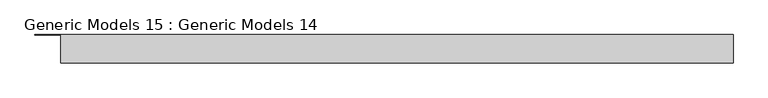
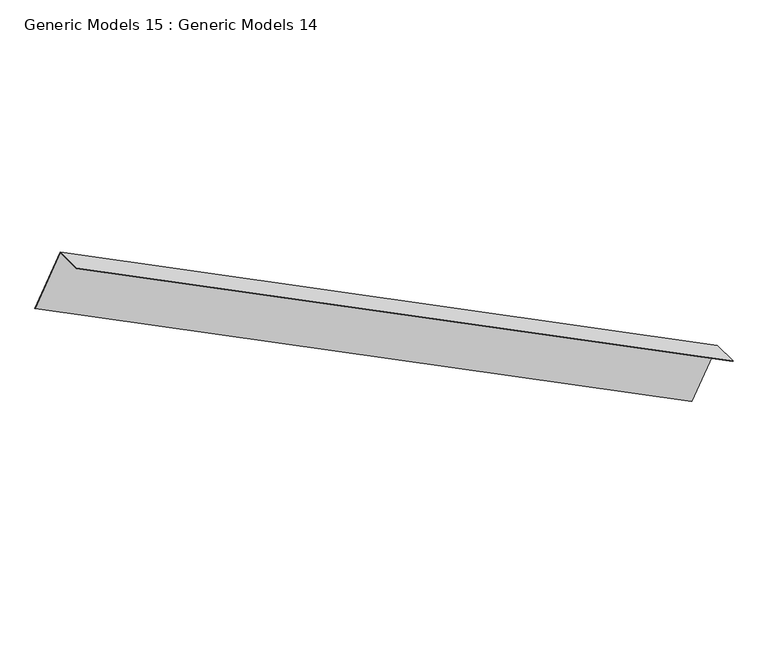
"""IFC4 building model written with IfcOpenShell, lengths in millimetres: proxy geometry, Generic Models 15 : Generic Models 14."""

from ifc_helpers import new_model, si_unit, frame, origin, place, context, project, spatial, polyline, outline, extrude, source, transform, mapped, element, save


def generic_models_15_generic_models_14_36b141fe(model_context):
    return source(origin(), model_context, "Body", "SweptSolid", [
        extrude(outline(polyline([(359.2115597, 0.0), (359.2115597, -1.5875), (-1.5875, -1.5875), (-1.5875, 175.4370114), (0.0, 175.4370114), (0.0, 0.0), (359.2115597, 0.0)])), frame((32076.3023425, 40953.6089828, 272263.2749093), z_axis=(-0.8944271909999191, 0.0, 0.44721359549995154), x_axis=(-0.44721359549995154, 0.0, -0.8944271909999191)), (0.0, 0.0, 1.0), 4676.5930666),
    ])


if __name__ == "__main__":
    model = new_model("IFC4")
    model_context = context("Model", 3, world=origin())
    ifc_project = project(units=[si_unit("LENGTHUNIT", "METRE", prefix="MILLI")], contexts=[model_context])
    site = spatial("IfcSite", under=ifc_project)
    building = spatial("IfcBuilding", under=site)
    placement = place(None, origin())
    generic_models_15_generic_models_14_shape = generic_models_15_generic_models_14_36b141fe(model_context)
    element("IfcBuildingElementProxy", 1, Name="Generic Models 15 : Generic Models 14", ObjectType="Generic Models 15 : Generic Models 14", at=placement, inside=building, context=model_context, shape_type="MappedRepresentation", body=[
        mapped(generic_models_15_generic_models_14_shape, transform((0.0, 0.0, 0.0), x_axis=(1.0, 0.0, 0.0), y_axis=(0.0, 1.0, 0.0), z_axis=(0.0, 0.0, 1.0))),
    ])
    save(model, "model.ifc")

# Revit data of these elements
# Element 1 (IfcBuildingElementProxy, "Generic Models 15 : Generic Models 14")
#   Materials on its faces: "EXTEND UV STABLE (WRVPAB) OVER ROOF SHEATHING - UNDER ROOF FELT"
# Materials
#   "EXTEND UV STABLE (WRVPAB) OVER ROOF SHEATHING - UNDER ROOF FELT": class "Unassigned", colour RGB 255 255 255, transparency 0, Cost = 0
